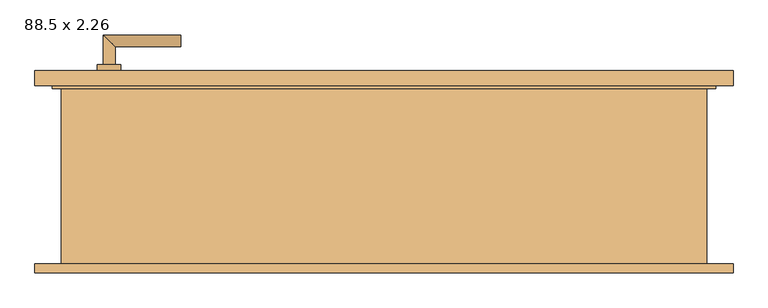
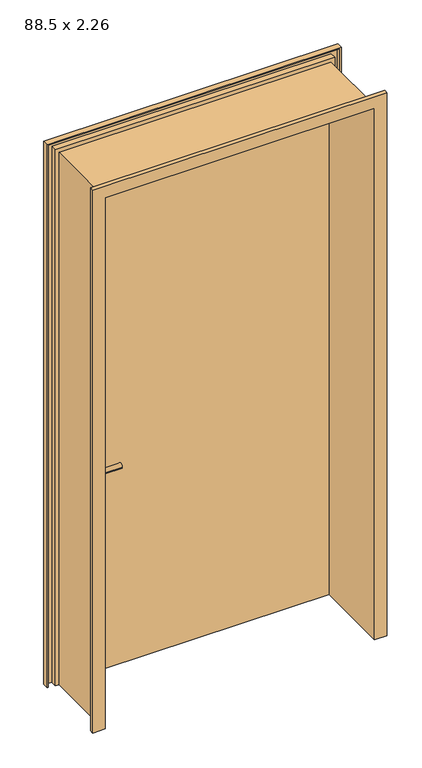
"""IFC4 building model written with IfcOpenShell, lengths in millimetres: door geometry, Drehflügel 1-flg - Stahlzarge : 88.5 x 2.26."""

import ifcopenshell
import ifcopenshell.guid

model = None  # the IFC model being written
_history = None  # IfcOwnerHistory: only IFC2X3 demands one
_inside = {}  # id of a spatial element -> (the spatial element, [elements in it])
_under = {}  # id of a project, library or spatial element -> (it, [spatial elements below it])
_declared = {}  # id of a project -> (the project, [libraries it declares])
_typed = {}  # id of a type object -> (the type object, [elements of that type])
_made_of = {}  # id of a material, layer set ... -> (it, [elements and type objects made of it])


def new_model(schema):
    """Start an empty IFC model of exactly this schema.

    Asked for "IFC4X3", IfcOpenShell would pick the latest addendum, in which some entities
    have other attributes; the version numbers below select the first issue.
    IFC2X3 requires an IfcOwnerHistory on every rooted entity: one is made here for all.
    """
    global model, _history
    if schema == "IFC4X3":
        model = ifcopenshell.file(schema_version=(4, 3, 0, 0))
    else:
        model = ifcopenshell.file(schema=schema)
    _inside.clear()
    _under.clear()
    _declared.clear()
    _typed.clear()
    _made_of.clear()
    _history = None
    if model.schema == "IFC2X3":
        org = make("IfcOrganization", Name="unknown")
        user = make(
            "IfcPersonAndOrganization",
            ThePerson=make("IfcPerson", FamilyName="unknown"),
            TheOrganization=org,
        )
        app = make(
            "IfcApplication",
            ApplicationDeveloper=org,
            Version="unknown",
            ApplicationFullName="unknown",
            ApplicationIdentifier="unknown",
        )
        _history = make(
            "IfcOwnerHistory",
            OwningUser=user,
            OwningApplication=app,
            ChangeAction="ADDED",
            CreationDate=0,
        )
    return model


def make(cls, **values):
    """One entity of the class cls with the attributes given. An attribute that is None is left unset."""
    return model.create_entity(
        cls, **{name: value for name, value in values.items() if value is not None}
    )


def rooted(cls, **values):
    """An entity with a GlobalId (a new one), such as an element, a storey or a relation."""
    return make(cls, GlobalId=ifcopenshell.guid.new(), OwnerHistory=_history, **values)


def si_unit(unit_type, name, prefix=None):
    """IfcSIUnit, for example si_unit("LENGTHUNIT", "METRE", prefix="MILLI")."""
    return make("IfcSIUnit", UnitType=unit_type, Prefix=prefix, Name=name)


def assignment(units):
    """IfcUnitAssignment: the units of a project."""
    return None if units is None else make("IfcUnitAssignment", Units=units)


def point(xyz):
    """IfcCartesianPoint."""
    return None if xyz is None else make("IfcCartesianPoint", Coordinates=xyz)


def direction(xyz):
    """IfcDirection."""
    return None if xyz is None else make("IfcDirection", DirectionRatios=xyz)


def frame(location, z_axis=None, x_axis=None):
    """IfcAxis2Placement3D, a coordinate frame: its origin and axes. An axis left out is left unset."""
    return make(
        "IfcAxis2Placement3D",
        Location=point(location),
        Axis=direction(z_axis),
        RefDirection=direction(x_axis),
    )


def frame_2d(location, x_axis=None):
    """IfcAxis2Placement2D, a coordinate frame in the plane: its origin and x axis."""
    return make(
        "IfcAxis2Placement2D", Location=point(location), RefDirection=direction(x_axis)
    )


def origin():
    """The frame at (0, 0, 0) with its axes left unset."""
    return frame((0.0, 0.0, 0.0))


def place(relative_to, where):
    """IfcLocalPlacement: puts the frame where relative to a parent placement (None: the world)."""
    return make(
        "IfcLocalPlacement", PlacementRelTo=relative_to, RelativePlacement=where
    )


def context(
    kind, dimensions, precision=None, world=None, true_north=None, identifier=None
):
    """IfcGeometricRepresentationContext, for example the 3D "Model" context."""
    return make(
        "IfcGeometricRepresentationContext",
        ContextIdentifier=identifier,
        ContextType=kind,
        CoordinateSpaceDimension=dimensions,
        Precision=precision,
        WorldCoordinateSystem=world,
        TrueNorth=true_north,
    )


def project(units=None, contexts=None):
    """IfcProject with its units and contexts."""
    return rooted(
        "IfcProject",
        Name="project",
        RepresentationContexts=contexts,
        UnitsInContext=assignment(units),
    )


def spatial(cls, under=None, at=None, **own):
    """A site, building, storey or space (cls), placed at a placement, below another one or the project."""
    s = rooted(cls, ObjectPlacement=at, **own)
    if under is not None:
        _under.setdefault(under.id(), (under, []))[1].append(s)
    return s


def polyline(points):
    """IfcPolyline through the points."""
    return make("IfcPolyline", Points=[point(p) for p in points])


def circle_curve(where, radius):
    """IfcCircle in the frame where."""
    return make("IfcCircle", Position=where, Radius=radius)


def ellipse_curve(where, semi_axis1, semi_axis2):
    """IfcEllipse in the frame where."""
    return make(
        "IfcEllipse", Position=where, SemiAxis1=semi_axis1, SemiAxis2=semi_axis2
    )


def trimmed(basis, trim1, trim2, sense, master):
    """IfcTrimmedCurve: the piece of a basis curve between two trims."""
    return make(
        "IfcTrimmedCurve",
        BasisCurve=basis,
        Trim1=trim1,
        Trim2=trim2,
        SenseAgreement=sense,
        MasterRepresentation=master,
    )


def segment(curve, same_sense, transition):
    """IfcCompositeCurveSegment."""
    return make(
        "IfcCompositeCurveSegment",
        Transition=transition,
        SameSense=same_sense,
        ParentCurve=curve,
    )


def composite_curve(segments, self_intersect=None):
    """IfcCompositeCurve: segments joined end to end."""
    return make("IfcCompositeCurve", Segments=segments, SelfIntersect=self_intersect)


def outline(outer, holes=None, kind="AREA"):
    """IfcArbitraryClosedProfileDef: a profile drawn as a closed curve; with holes, ...WithVoids."""
    if holes is None:
        return make("IfcArbitraryClosedProfileDef", ProfileType=kind, OuterCurve=outer)
    return make(
        "IfcArbitraryProfileDefWithVoids",
        ProfileType=kind,
        OuterCurve=outer,
        InnerCurves=holes,
    )


def extrude(swept, where, along, depth):
    """IfcExtrudedAreaSolid: the profile swept, set in the frame where, extruded along a direction by depth."""
    return make(
        "IfcExtrudedAreaSolid",
        SweptArea=swept,
        Position=where,
        ExtrudedDirection=direction(along),
        Depth=depth,
    )


def faces_of(points, faces, orient=None, outer=None):
    """IfcFace entities. A face is a list of loops; a loop is a list of indices into points, from 0.

    orient and outer hold one flag for each loop. By default every Orientation is true, the
    first loop of a face is its IfcFaceOuterBound and the others are IfcFaceBound.
    """
    made = []
    for i, loops in enumerate(faces):
        bounds = []
        for j, loop in enumerate(loops):
            is_outer = j == 0 if outer is None else outer[i][j]
            bounds.append(
                make(
                    "IfcFaceOuterBound" if is_outer else "IfcFaceBound",
                    Bound=make("IfcPolyLoop", Polygon=[points[k] for k in loop]),
                    Orientation=True if orient is None else orient[i][j],
                )
            )
        made.append(make("IfcFace", Bounds=bounds))
    return made


def faceted_brep(points, faces, orient=None, outer=None, voids=None):
    """IfcFacetedBrep: a solid bounded by flat faces; with voids (closed shells), ...WithVoids."""
    shared = [point(p) for p in points]
    hull = make("IfcClosedShell", CfsFaces=faces_of(shared, faces, orient, outer))
    if voids is None:
        return make("IfcFacetedBrep", Outer=hull)
    return make(
        "IfcFacetedBrepWithVoids",
        Outer=hull,
        Voids=[
            make(cls, CfsFaces=faces_of(shared, fs, o, b)) for cls, fs, o, b in voids
        ],
    )


def shape(context_of_items, identifier, shape_type, items):
    """IfcShapeRepresentation: the items that make up one representation, for example the "Body"."""
    return make(
        "IfcShapeRepresentation",
        ContextOfItems=context_of_items,
        RepresentationIdentifier=identifier,
        RepresentationType=shape_type,
        Items=items,
    )


def source(mapping_origin, context_of_items, identifier, shape_type, items):
    """IfcRepresentationMap: a shape defined once, which mapped items show again and again."""
    return make(
        "IfcRepresentationMap",
        MappingOrigin=mapping_origin,
        MappedRepresentation=shape(context_of_items, identifier, shape_type, items),
    )


def transform(
    local_origin,
    x_axis=None,
    y_axis=None,
    z_axis=None,
    scale=None,
    scale2=None,
    scale3=None,
    uniform=True,
):
    """IfcCartesianTransformationOperator3D, or its non-uniform kind. x_axis, y_axis, z_axis: its Axis1, 2, 3."""
    if uniform:
        return make(
            "IfcCartesianTransformationOperator3D",
            Axis1=direction(x_axis),
            Axis2=direction(y_axis),
            LocalOrigin=point(local_origin),
            Scale=scale,
            Axis3=direction(z_axis),
        )
    return make(
        "IfcCartesianTransformationOperator3DnonUniform",
        Axis1=direction(x_axis),
        Axis2=direction(y_axis),
        LocalOrigin=point(local_origin),
        Scale=scale,
        Axis3=direction(z_axis),
        Scale2=scale2,
        Scale3=scale3,
    )


def mapped(mapping_source, mapping_target):
    """IfcMappedItem: shows the shape of a source again, moved by a transform."""
    return make(
        "IfcMappedItem", MappingSource=mapping_source, MappingTarget=mapping_target
    )


def made_of(thing, what):
    """Note that an element or type object is made of a material, layer set ...; save() writes the relation."""
    if what is not None:
        _made_of.setdefault(what.id(), (what, []))[1].append(thing)
    return thing


def element(
    cls,
    number,
    at=None,
    inside=None,
    cuts=None,
    type_object=None,
    material=None,
    context=None,
    identifier="Body",
    shape_type=None,
    held_by="IfcProductDefinitionShape",
    body=None,
    shapes=None,
    **own,
):
    """One element of the class cls, such as IfcWall. Its Tag is "e" and its number.

    at: its placement. inside: the storey or other place that contains it. cuts: it is an
    opening in that element (IfcRelVoidsElement). A single representation is given by context,
    identifier, shape_type and body (its items); several are given by shapes. held_by: the class
    of the entity that holds the representations. save() writes the other relations.
    """
    e = rooted(cls, Tag="e%d" % number, ObjectPlacement=at, **own)
    if body is not None:
        shapes = [shape(context, identifier, shape_type, body)]
    if shapes is not None:
        e.Representation = make(held_by, Representations=shapes)
    if inside is not None:
        _inside.setdefault(inside.id(), (inside, []))[1].append(e)
    if cuts is not None:
        rooted(
            "IfcRelVoidsElement", RelatingBuildingElement=cuts, RelatedOpeningElement=e
        )
    if type_object is not None:
        _typed.setdefault(type_object.id(), (type_object, []))[1].append(e)
    return made_of(e, material)


def aggregate(whole, parts):
    """IfcRelAggregates: a whole, such as a stair, and the parts it consists of."""
    return rooted("IfcRelAggregates", RelatingObject=whole, RelatedObjects=parts)


def save(model, path):
    """Write the relations noted so far, then the file.

    IfcRelAggregates (storeys below a building ...), IfcRelContainedInSpatialStructure (elements
    in a storey), IfcRelDefinesByType, IfcRelAssociatesMaterial and IfcRelDeclares: one each for
    every whole, place, type object, material and project.
    """
    for whole, parts in _under.values():
        aggregate(whole, parts)
    for where, things in _inside.values():
        rooted(
            "IfcRelContainedInSpatialStructure",
            RelatedElements=things,
            RelatingStructure=where,
        )
    for kind, things in _typed.values():
        rooted("IfcRelDefinesByType", RelatedObjects=things, RelatingType=kind)
    for what, things in _made_of.values():
        rooted("IfcRelAssociatesMaterial", RelatedObjects=things, RelatingMaterial=what)
    for by, libraries in _declared.values():
        rooted("IfcRelDeclares", RelatingContext=by, RelatedDefinitions=libraries)
    model.write(path)


def plane_surface(at):
    """IfcPlane: the flat surface through the origin of the frame at, square to its z axis."""
    return make("IfcPlane", Position=at)


def cylinder_surface(at, radius):
    """IfcCylindricalSurface: all points at the distance radius from the z axis of the frame at."""
    return make("IfcCylindricalSurface", Position=at, Radius=radius)


def advanced_brep(points, edges, surfaces, faces):
    """IfcAdvancedBrep: a solid bounded by faces that lie on surfaces and meet in shared edges.

    An edge is (start, end): straight between two places in points (the first is 0);
    or (start, end, curve); or (start, end, curve, False) where it runs against its curve.
    A face is (place in surfaces, loops), or (place, loops, False) where it looks against
    its surface's normal. A loop lists edges by number (the first is 1), with a minus sign
    where the edge is run from its end to its start. The first loop is the outer one.
    """
    corners = [point(p) for p in points]
    vertices = [make("IfcVertexPoint", VertexGeometry=c) for c in corners]
    made = []
    for start, end, *more in edges:
        made.append(
            make(
                "IfcEdgeCurve",
                EdgeStart=vertices[start],
                EdgeEnd=vertices[end],
                EdgeGeometry=more[0] if more else make("IfcPolyline", Points=[corners[start], corners[end]]),
                SameSense=more[1] if len(more) > 1 else True,
            )
        )
    hull = []
    for where, loops, *sense in faces:
        bounds = []
        for j, loop in enumerate(loops):
            ring = [make("IfcOrientedEdge", EdgeElement=made[abs(k) - 1], Orientation=k > 0) for k in loop]
            bounds.append(
                make(
                    "IfcFaceOuterBound" if j == 0 else "IfcFaceBound",
                    Bound=make("IfcEdgeLoop", EdgeList=ring),
                    Orientation=True,
                )
            )
        hull.append(make("IfcAdvancedFace", Bounds=bounds, FaceSurface=surfaces[where], SameSense=sense[0] if sense else True))
    return make("IfcAdvancedBrep", Outer=make("IfcClosedShell", CfsFaces=hull))


def door_88_5_x_2_26_3ccb849c(model_context):
    return source(origin(), model_context, "Body", "SolidModel", [
        advanced_brep(
        [(-471.4, 139.4346141, 1000.0), (-451.4, 139.4346141, 1000.0), (-471.4, 69.4346141, 1000.0), (-451.4, 89.4346141, 1000.0), (-341.4, 69.4346141, 1000.0), (-341.4, 89.4346141, 1000.0)],
        [
            (0, 1, circle_curve(frame((-461.4, 139.4346141, 1000.0), z_axis=(0.0, 1.0, 0.0), x_axis=(1.0, 0.0, 0.0)), 10.0)),
            (1, 0, circle_curve(frame((-461.4, 139.4346141, 1000.0), z_axis=(0.0, 1.0, 0.0), x_axis=(1.0, 0.0, 0.0)), 10.0)),
            (0, 2),
            (2, 3, ellipse_curve(frame((-461.4, 79.4346141, 1000.0), z_axis=(-0.7071067811865385, 0.7071067811865565, 0.0), x_axis=(0.7071067811865563, 0.7071067811865386, 0.0)), 14.1421356, 10.0)),
            (3, 1),
            (3, 2, ellipse_curve(frame((-461.4, 79.4346141, 1000.0), z_axis=(-0.7071067811865385, 0.7071067811865565, 0.0), x_axis=(0.7071067811865563, 0.7071067811865386, 0.0)), 14.1421356, 10.0)),
            (4, 5, circle_curve(frame((-341.4, 79.4346141, 1000.0), z_axis=(1.0, 0.0, 0.0), x_axis=(0.0, 1.0, 0.0)), 10.0)),
            (5, 4, circle_curve(frame((-341.4, 79.4346141, 1000.0), z_axis=(1.0, 0.0, 0.0), x_axis=(0.0, 1.0, 0.0)), 10.0)),
            (2, 4),
            (5, 3),
        ],
        [
            plane_surface(frame((-461.4, 139.4346141, -287.7526403), z_axis=(0.0, 1.0, 0.0), x_axis=(0.0, 0.0, 1.0))),
            cylinder_surface(frame((-461.4, 139.4346141, 1000.0), z_axis=(0.0, 1.0, 0.0), x_axis=(1.0, 0.0, 0.0)), 10.0),
            plane_surface(frame((-341.4, 79.4346141, -287.7526403), z_axis=(1.0, 0.0, 0.0), x_axis=(0.0, 0.0, 1.0))),
            cylinder_surface(frame((-461.4, 79.4346141, 1000.0), z_axis=(-1.0, 0.0, 0.0), x_axis=(0.0, 1.0, 0.0)), 10.0),
        ],
        [
            (0, [[1, 2]]),
            (1, [[-1, 3, 4, 5]]),
            (1, [[-2, -5, 6, -3]]),
            (2, [[7, 8]]),
            (3, [[-4, 9, -8, 10]]),
            (3, [[-6, -10, -7, -9]]),
        ],
    ),
        advanced_brep(
        [(-451.4, 199.4346141, 1000.0), (-471.4, 199.4346141, 1000.0), (-451.4, 229.4346141, 1000.0), (-471.4, 249.4346141, 1000.0), (-341.4, 229.4346141, 1000.0), (-341.4, 249.4346141, 1000.0)],
        [
            (0, 1, circle_curve(frame((-461.4, 199.4346141, 1000.0), z_axis=(0.0, -1.0, 0.0), x_axis=(-1.0, 0.0, 0.0)), 10.0)),
            (1, 0, circle_curve(frame((-461.4, 199.4346141, 1000.0), z_axis=(0.0, -1.0, 0.0), x_axis=(-1.0, 0.0, 0.0)), 10.0)),
            (0, 2),
            (2, 3, ellipse_curve(frame((-461.4, 239.4346141, 1000.0), z_axis=(-0.7071067811865475, -0.7071067811865475, 0.0), x_axis=(0.7071067811865474, -0.7071067811865476, 0.0)), 14.1421356, 10.0)),
            (3, 1),
            (3, 2, ellipse_curve(frame((-461.4, 239.4346141, 1000.0), z_axis=(-0.7071067811865475, -0.7071067811865475, 0.0), x_axis=(0.7071067811865474, -0.7071067811865476, 0.0)), 14.1421356, 10.0)),
            (4, 5, circle_curve(frame((-341.4, 239.4346141, 1000.0), z_axis=(1.0, 0.0, 0.0), x_axis=(0.0, 1.0, 0.0)), 10.0)),
            (5, 4, circle_curve(frame((-341.4, 239.4346141, 1000.0), z_axis=(1.0, 0.0, 0.0), x_axis=(0.0, 1.0, 0.0)), 10.0)),
            (2, 4),
            (5, 3),
        ],
        [
            plane_surface(frame((-461.4, 199.4346141, -287.7526403), z_axis=(0.0, -1.0, 0.0), x_axis=(0.0, 0.0, 1.0))),
            cylinder_surface(frame((-461.4, 199.4346141, 1000.0), z_axis=(0.0, -1.0, 0.0), x_axis=(-1.0, 0.0, 0.0)), 10.0),
            plane_surface(frame((-341.4, 239.4346141, -287.7526403), z_axis=(1.0, 0.0, 0.0), x_axis=(0.0, 0.0, 1.0))),
            cylinder_surface(frame((-461.4, 239.4346141, 1000.0), z_axis=(-1.0, 0.0, 0.0), x_axis=(0.0, 1.0, 0.0)), 10.0),
        ],
        [
            (0, [[1, 2]]),
            (1, [[-1, 3, 4, 5]]),
            (1, [[-2, -5, 6, -3]]),
            (2, [[7, 8]]),
            (3, [[-4, 9, -8, 10]]),
            (3, [[-6, -10, -7, -9]]),
        ],
    ),
        extrude(outline(composite_curve([segment(trimmed(circle_curve(frame_2d((1000.0, -461.4)), 20.0), [point((1000.0, -481.4))], [point((1000.0, -441.4))], False, "CARTESIAN"), True, "CONTINUOUS"), segment(trimmed(circle_curve(frame_2d((1000.0, -461.4)), 20.0), [point((1000.0, -441.4))], [point((1000.0, -481.4))], False, "CARTESIAN"), True, "CONTINUOUS")], self_intersect=False)), frame((0.0, 129.4346141, 0.0), z_axis=(0.0, 1.0, 0.0), x_axis=(0.0, 0.0, 1.0)), (0.0, 0.0, 1.0), 10.0),
        extrude(outline(composite_curve([segment(trimmed(circle_curve(frame_2d((1000.0, -461.4)), 20.0), [point((1000.0, -481.4))], [point((1000.0, -441.4))], False, "CARTESIAN"), True, "CONTINUOUS"), segment(trimmed(circle_curve(frame_2d((1000.0, -461.4)), 20.0), [point((1000.0, -441.4))], [point((1000.0, -481.4))], False, "CARTESIAN"), True, "CONTINUOUS")], self_intersect=False)), frame((0.0, 189.4346141, 0.0), z_axis=(0.0, 1.0, 0.0), x_axis=(0.0, 0.0, 1.0)), (0.0, 0.0, 1.0), 10.0),
        extrude(outline(polyline([(551.4, 164.4346141), (-551.4, 164.4346141), (-551.4, 189.4346141), (551.4, 189.4346141), (551.4, 164.4346141)])), frame((0.0, 0.0, 100.0), z_axis=(0.0, 0.0, 1.0), x_axis=(1.0, 0.0, 0.0)), (0.0, 0.0, 1.0), 2250.0),
        faceted_brep([(585.8603207, -150.5653859, 100.0), (536.4, -150.5653859, 100.0), (536.4, 164.4346141, 100.0), (551.4, 164.4346141, 100.0), (551.4, 189.4346141, 100.0), (585.8603207, 189.4346141, 100.0), (585.8603207, 164.4346141, 100.0), (580.8603207, 164.4346141, 100.0), (580.8603207, 184.4346141, 100.0), (556.4, 184.4346141, 100.0), (556.4, 159.4346141, 100.0), (541.4, 159.4346141, 100.0), (541.4, -145.5653859, 100.0), (580.8603207, -145.5653859, 100.0), (580.8603207, -135.5653859, 100.0), (585.8603207, -135.5653859, 100.0), (585.8603207, -150.5653859, 2384.4603207), (-585.8603207, -150.5653859, 2384.4603207), (-585.8603207, -150.5653859, 100.0), (-536.4, -150.5653859, 100.0), (-536.4, -150.5653859, 2335.0), (536.4, -150.5653859, 2335.0), (536.4, 164.4346141, 2335.0), (-536.4, 164.4346141, 2335.0), (-536.4, 164.4346141, 100.0), (-551.4, 164.4346141, 100.0), (-551.4, 164.4346141, 2350.0), (551.4, 164.4346141, 2350.0), (551.4, 189.4346141, 2350.0), (-551.4, 189.4346141, 2350.0), (-551.4, 189.4346141, 100.0), (-585.8603207, 189.4346141, 100.0), (-585.8603207, 189.4346141, 2384.4603207), (585.8603207, 189.4346141, 2384.4603207), (585.8603207, 164.4346141, 2384.4603207), (-585.8603207, 164.4346141, 2384.4603207), (-585.8603207, 164.4346141, 100.0), (-580.8603207, 164.4346141, 100.0), (-580.8603207, 164.4346141, 2379.4603207), (580.8603207, 164.4346141, 2379.4603207), (580.8603207, 184.4346141, 2379.4603207), (-580.8603207, 184.4346141, 2379.4603207), (-580.8603207, 184.4346141, 100.0), (-556.4, 184.4346141, 100.0), (-556.4, 184.4346141, 2355.0), (556.4, 184.4346141, 2355.0), (556.4, 159.4346141, 2355.0), (-556.4, 159.4346141, 2355.0), (-556.4, 159.4346141, 100.0), (-541.4, 159.4346141, 100.0), (-541.4, 159.4346141, 2340.0), (541.4, 159.4346141, 2340.0), (541.4, -145.5653859, 2340.0), (-541.4, -145.5653859, 2340.0), (-541.4, -145.5653859, 100.0), (-580.8603207, -145.5653859, 100.0), (-580.8603207, -145.5653859, 2379.4603207), (580.8603207, -145.5653859, 2379.4603207), (580.8603207, -135.5653859, 2379.4603207), (-580.8603207, -135.5653859, 2379.4603207), (-580.8603207, -135.5653859, 100.0), (-585.8603207, -135.5653859, 100.0), (-585.8603207, -135.5653859, 2384.4603207), (585.8603207, -135.5653859, 2384.4603207)], [[[0, 1, 2, 3, 4, 5, 6, 7, 8, 9, 10, 11, 12, 13, 14, 15]], [[1, 0, 16, 17, 18, 19, 20, 21]], [[2, 1, 21, 22]], [[3, 2, 22, 23, 24, 25, 26, 27]], [[4, 3, 27, 28]], [[5, 4, 28, 29, 30, 31, 32, 33]], [[6, 5, 33, 34]], [[7, 6, 34, 35, 36, 37, 38, 39]], [[8, 7, 39, 40]], [[9, 8, 40, 41, 42, 43, 44, 45]], [[10, 9, 45, 46]], [[11, 10, 46, 47, 48, 49, 50, 51]], [[12, 11, 51, 52]], [[13, 12, 52, 53, 54, 55, 56, 57]], [[14, 13, 57, 58]], [[15, 14, 58, 59, 60, 61, 62, 63]], [[0, 15, 63, 16]], [[17, 62, 61, 18]], [[18, 61, 60, 55, 54, 49, 48, 43, 42, 37, 36, 31, 30, 25, 24, 19]], [[23, 20, 19, 24]], [[29, 26, 25, 30]], [[35, 32, 31, 36]], [[41, 38, 37, 42]], [[47, 44, 43, 48]], [[53, 50, 49, 54]], [[59, 56, 55, 60]], [[22, 21, 20, 23]], [[28, 27, 26, 29]], [[34, 33, 32, 35]], [[40, 39, 38, 41]], [[46, 45, 44, 47]], [[52, 51, 50, 53]], [[58, 57, 56, 59]], [[16, 63, 62, 17]]]),
    ])


if __name__ == "__main__":
    model = new_model("IFC4")
    model_context = context("Model", 3, world=origin())
    ifc_project = project(units=[si_unit("LENGTHUNIT", "METRE", prefix="MILLI")], contexts=[model_context])
    site = spatial("IfcSite", under=ifc_project)
    building = spatial("IfcBuilding", under=site)
    placement = place(None, origin())
    door_88_5_x_2_26_shape = door_88_5_x_2_26_3ccb849c(model_context)
    element("IfcDoor", 1, ObjectType="Drehflügel 1-flg - Stahlzarge : 88.5 x 2.26", at=placement, inside=building, context=model_context, shape_type="MappedRepresentation", body=[
        mapped(door_88_5_x_2_26_shape, transform((0.0, 0.0, 0.0), x_axis=(1.0, 0.0, 0.0), y_axis=(0.0, 1.0, 0.0), z_axis=(0.0, 0.0, 1.0))),
    ])
    save(model, "model.ifc")

# Revit data of these elements
# Type "Drehflügel 1-flg - Stahlzarge : 88.5 x 2.26"
#   Construction Type Id = "MDOOR"
#   Type Mark = "20"
#   Operation = "SingleSwingRight"
#   Keynote = "16.03"
#   Analytic Construction = "Metall"
#   Thermal Resistance (R) = 0.270117 (m²·K)/W
#   Heat Transfer Coefficient (U) = 3.7021 W/(m²·K)
#   Rough Width = 1.1228 m
#   Rough Height [instance default] = 2.360 m
#   Höhe Türgriff [instance default] = 0.900 m
#   Height = 2.260 m
#   Fußbodenaufbau [instance default] = 0.100 m
#   Width = 1.1228 m
#   Sichtbarkeit Sturzlinien [instance default] = yes
#   Türgriff auswählen [instance default] = element 221079
#   Türgriff [instance default] = none
#   Türflügel [instance default] = none
#   Rahmen/Pfosten [instance default] = Metall - Lackiert - Grau
#   Visual Light Transmittance = 0
#   Solar Heat Gain Coefficient = 0
#   Function = (empty or 0)
#   Wall Closure = (empty or 0)
# Element 1 (IfcDoor, "Drehflügel 1-flg - Stahlzarge : 88.5 x 2.26")
#   Materials on its faces: "Metall - Lackiert - Grau", "Metall - Chrom", "Holz - Birke"
# Materials
#   "Metall - Lackiert - Grau": class "Farbe 1", colour RGB 98 98 98, transparency 0, Cost = 0
#   "Metall - Chrom": class "Metall", colour RGB 247 247 247, transparency 0, Cost = 0
#   "Holz - Birke": class "Holz", colour RGB 213 164 103, transparency 0, Cost = 0
